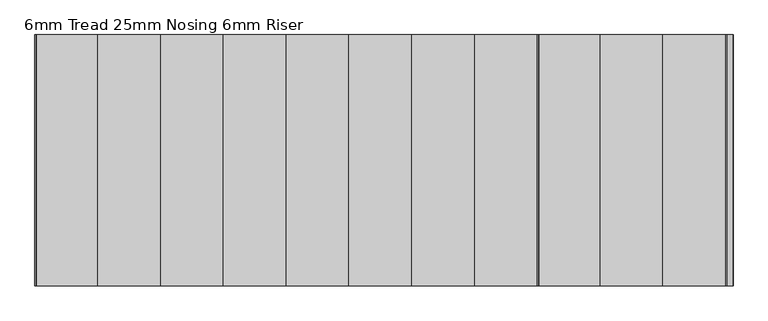
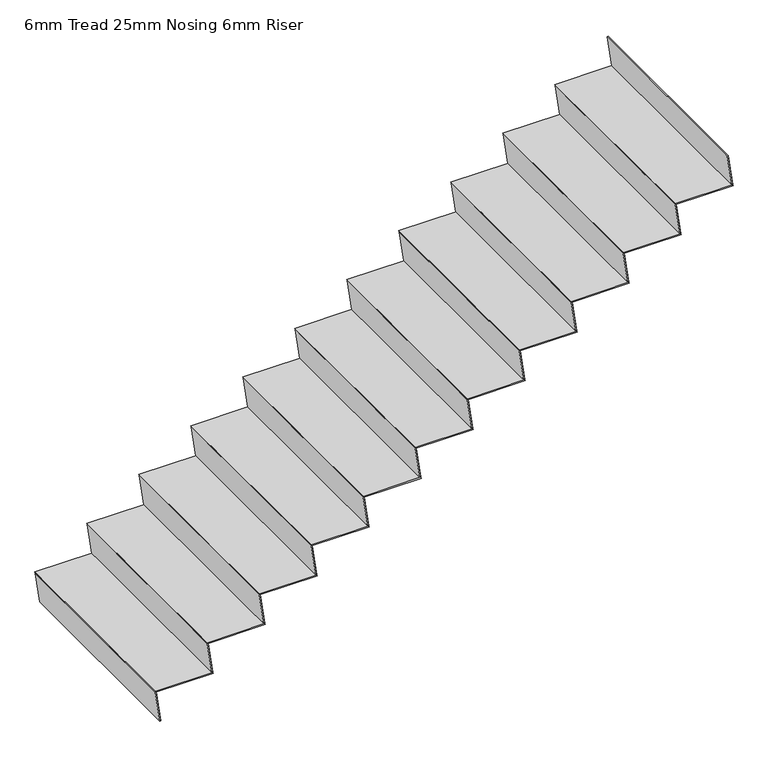
"""IFC4 building model written with IfcOpenShell, lengths in millimetres: stair flight geometry, 6mm Tread 25mm Nosing 6mm Riser."""

from ifc_helpers import new_model, si_unit, origin, place, context, project, spatial, faceted_brep, source, transform, mapped, element, save


def stair_flight_6mm_tread_25mm_nosing_6mm_riser_6b1513e0(model_context):
    return source(origin(), model_context, "Body", "Brep", [
        faceted_brep([(-16043.9400908, 12075.4345331, 22294.1176471), (-16043.0900908, 12075.4345331, 22288.1176471), (-16043.0900908, 13175.4345331, 22288.1176471), (-16043.9400908, 13175.4345331, 22294.1176471), (-16350.0, 13175.4345331, 22294.1176471), (-16350.0, 12075.4345331, 22294.1176471), (-16349.15, 12075.4345331, 22288.1176471), (-16349.15, 13175.4345331, 22288.1176471)], [[[0, 1, 2, 3]], [[3, 4, 5, 0]], [[2, 1, 6, 7]], [[4, 3, 2, 7]], [[0, 5, 6, 1]], [[5, 4, 7, 6]]]),
        faceted_brep([(-16349.15, 12075.4345331, 22288.1176471), (-16325.0, 12075.4345331, 22117.6470588), (-16318.9400908, 12075.4345331, 22117.6470588), (-16343.0900908, 12075.4345331, 22288.1176471), (-16349.15, 13175.4345331, 22288.1176471), (-16343.0900908, 13175.4345331, 22288.1176471), (-16318.9400908, 13175.4345331, 22117.6470588), (-16325.0, 13175.4345331, 22117.6470588)], [[[0, 1, 2, 3]], [[4, 5, 6, 7]], [[1, 0, 4, 7]], [[2, 1, 7, 6]], [[3, 2, 6, 5]], [[0, 3, 5, 4]]]),
        faceted_brep([(-16074.15, 12075.4345331, 22464.5882353), (-16050.0, 12075.4345331, 22294.1176471), (-16043.9400908, 12075.4345331, 22294.1176471), (-16068.0900908, 12075.4345331, 22464.5882353), (-16074.15, 13175.4345331, 22464.5882353), (-16068.0900908, 13175.4345331, 22464.5882353), (-16043.9400908, 13175.4345331, 22294.1176471), (-16050.0, 13175.4345331, 22294.1176471)], [[[0, 1, 2, 3]], [[4, 5, 6, 7]], [[1, 0, 4, 7]], [[2, 1, 7, 6]], [[3, 2, 6, 5]], [[0, 3, 5, 4]]]),
        faceted_brep([(-15768.9400908, 13175.4345331, 22470.5882353), (-16075.0, 13175.4345331, 22470.5882353), (-16075.0, 12075.4345331, 22470.5882353), (-15768.9400908, 12075.4345331, 22470.5882353), (-15768.0900908, 13175.4345331, 22464.5882353), (-15768.0900908, 12075.4345331, 22464.5882353), (-16074.15, 12075.4345331, 22464.5882353), (-16074.15, 13175.4345331, 22464.5882353)], [[[0, 1, 2, 3]], [[4, 5, 6, 7]], [[1, 0, 4, 7]], [[3, 2, 6, 5]], [[3, 5, 4, 0]], [[2, 1, 7, 6]]]),
        faceted_brep([(-15799.15, 12075.4345331, 22641.0588235), (-15775.0, 12075.4345331, 22470.5882353), (-15768.9400908, 12075.4345331, 22470.5882353), (-15793.0900908, 12075.4345331, 22641.0588235), (-15799.15, 13175.4345331, 22641.0588235), (-15793.0900908, 13175.4345331, 22641.0588235), (-15768.9400908, 13175.4345331, 22470.5882353), (-15775.0, 13175.4345331, 22470.5882353)], [[[0, 1, 2, 3]], [[4, 5, 6, 7]], [[1, 0, 4, 7]], [[2, 1, 7, 6]], [[3, 2, 6, 5]], [[0, 3, 5, 4]]]),
        faceted_brep([(-15493.9400908, 13175.4345331, 22647.0588235), (-15800.0, 13175.4345331, 22647.0588235), (-15800.0, 12075.4345331, 22647.0588235), (-15493.9400908, 12075.4345331, 22647.0588235), (-15493.0900908, 13175.4345331, 22641.0588235), (-15493.0900908, 12075.4345331, 22641.0588235), (-15799.15, 12075.4345331, 22641.0588235), (-15799.15, 13175.4345331, 22641.0588235)], [[[0, 1, 2, 3]], [[4, 5, 6, 7]], [[1, 0, 4, 7]], [[3, 2, 6, 5]], [[3, 5, 4, 0]], [[2, 1, 7, 6]]]),
        faceted_brep([(-15524.15, 12075.4345331, 22817.5294118), (-15500.0, 12075.4345331, 22647.0588235), (-15493.9400908, 12075.4345331, 22647.0588235), (-15518.0900908, 12075.4345331, 22817.5294118), (-15524.15, 13175.4345331, 22817.5294118), (-15518.0900908, 13175.4345331, 22817.5294118), (-15493.9400908, 13175.4345331, 22647.0588235), (-15500.0, 13175.4345331, 22647.0588235)], [[[0, 1, 2, 3]], [[4, 5, 6, 7]], [[1, 0, 4, 7]], [[2, 1, 7, 6]], [[3, 2, 6, 5]], [[0, 3, 5, 4]]]),
        faceted_brep([(-15218.9400908, 13175.4345331, 22823.5294118), (-15525.0, 13175.4345331, 22823.5294118), (-15525.0, 12075.4345331, 22823.5294118), (-15218.9400908, 12075.4345331, 22823.5294118), (-15218.0900908, 13175.4345331, 22817.5294118), (-15218.0900908, 12075.4345331, 22817.5294118), (-15524.15, 12075.4345331, 22817.5294118), (-15524.15, 13175.4345331, 22817.5294118)], [[[0, 1, 2, 3]], [[4, 5, 6, 7]], [[1, 0, 4, 7]], [[3, 2, 6, 5]], [[3, 5, 4, 0]], [[2, 1, 7, 6]]]),
        faceted_brep([(-15249.15, 12075.4345331, 22994.0), (-15225.0, 12075.4345331, 22823.5294118), (-15218.9400908, 12075.4345331, 22823.5294118), (-15243.0900908, 12075.4345331, 22994.0), (-15249.15, 13175.4345331, 22994.0), (-15243.0900908, 13175.4345331, 22994.0), (-15218.9400908, 13175.4345331, 22823.5294118), (-15225.0, 13175.4345331, 22823.5294118)], [[[0, 1, 2, 3]], [[4, 5, 6, 7]], [[1, 0, 4, 7]], [[2, 1, 7, 6]], [[3, 2, 6, 5]], [[0, 3, 5, 4]]]),
        faceted_brep([(-14943.9400908, 13175.4345331, 23000.0), (-15250.0, 13175.4345331, 23000.0), (-15250.0, 12075.4345331, 23000.0), (-14943.9400908, 12075.4345331, 23000.0), (-14943.0900908, 13175.4345331, 22994.0), (-14943.0900908, 12075.4345331, 22994.0), (-15249.15, 12075.4345331, 22994.0), (-15249.15, 13175.4345331, 22994.0)], [[[0, 1, 2, 3]], [[4, 5, 6, 7]], [[1, 0, 4, 7]], [[3, 2, 6, 5]], [[3, 5, 4, 0]], [[2, 1, 7, 6]]]),
        faceted_brep([(-14974.15, 12075.4345331, 23170.4705882), (-14950.0, 12075.4345331, 23000.0), (-14943.9400908, 12075.4345331, 23000.0), (-14968.0900908, 12075.4345331, 23170.4705882), (-14974.15, 13175.4345331, 23170.4705882), (-14968.0900908, 13175.4345331, 23170.4705882), (-14943.9400908, 13175.4345331, 23000.0), (-14950.0, 13175.4345331, 23000.0)], [[[0, 1, 2, 3]], [[4, 5, 6, 7]], [[1, 0, 4, 7]], [[2, 1, 7, 6]], [[3, 2, 6, 5]], [[0, 3, 5, 4]]]),
        faceted_brep([(-14668.9400908, 13175.4345331, 23176.4705882), (-14975.0, 13175.4345331, 23176.4705882), (-14975.0, 12075.4345331, 23176.4705882), (-14668.9400908, 12075.4345331, 23176.4705882), (-14668.0900908, 13175.4345331, 23170.4705882), (-14668.0900908, 12075.4345331, 23170.4705882), (-14974.15, 12075.4345331, 23170.4705882), (-14974.15, 13175.4345331, 23170.4705882)], [[[0, 1, 2, 3]], [[4, 5, 6, 7]], [[1, 0, 4, 7]], [[3, 2, 6, 5]], [[3, 5, 4, 0]], [[2, 1, 7, 6]]]),
        faceted_brep([(-14699.15, 12075.4345331, 23346.9411765), (-14675.0, 12075.4345331, 23176.4705882), (-14668.9400908, 12075.4345331, 23176.4705882), (-14693.0900908, 12075.4345331, 23346.9411765), (-14699.15, 13175.4345331, 23346.9411765), (-14693.0900908, 13175.4345331, 23346.9411765), (-14668.9400908, 13175.4345331, 23176.4705882), (-14675.0, 13175.4345331, 23176.4705882)], [[[0, 1, 2, 3]], [[4, 5, 6, 7]], [[1, 0, 4, 7]], [[2, 1, 7, 6]], [[3, 2, 6, 5]], [[0, 3, 5, 4]]]),
        faceted_brep([(-14393.9400908, 13175.4345331, 23352.9411765), (-14700.0, 13175.4345331, 23352.9411765), (-14700.0, 12075.4345331, 23352.9411765), (-14393.9400908, 12075.4345331, 23352.9411765), (-14393.0900908, 13175.4345331, 23346.9411765), (-14393.0900908, 12075.4345331, 23346.9411765), (-14699.15, 12075.4345331, 23346.9411765), (-14699.15, 13175.4345331, 23346.9411765)], [[[0, 1, 2, 3]], [[4, 5, 6, 7]], [[1, 0, 4, 7]], [[3, 2, 6, 5]], [[3, 5, 4, 0]], [[2, 1, 7, 6]]]),
        faceted_brep([(-14424.15, 12075.4345331, 23523.4117647), (-14400.0, 12075.4345331, 23352.9411765), (-14393.9400908, 12075.4345331, 23352.9411765), (-14418.0900908, 12075.4345331, 23523.4117647), (-14424.15, 13175.4345331, 23523.4117647), (-14418.0900908, 13175.4345331, 23523.4117647), (-14393.9400908, 13175.4345331, 23352.9411765), (-14400.0, 13175.4345331, 23352.9411765)], [[[0, 1, 2, 3]], [[4, 5, 6, 7]], [[1, 0, 4, 7]], [[2, 1, 7, 6]], [[3, 2, 6, 5]], [[0, 3, 5, 4]]]),
        faceted_brep([(-14118.9400908, 13175.4345331, 23529.4117647), (-14425.0, 13175.4345331, 23529.4117647), (-14425.0, 12075.4345331, 23529.4117647), (-14118.9400908, 12075.4345331, 23529.4117647), (-14118.0900908, 13175.4345331, 23523.4117647), (-14118.0900908, 12075.4345331, 23523.4117647), (-14424.15, 12075.4345331, 23523.4117647), (-14424.15, 13175.4345331, 23523.4117647)], [[[0, 1, 2, 3]], [[4, 5, 6, 7]], [[1, 0, 4, 7]], [[3, 2, 6, 5]], [[3, 5, 4, 0]], [[2, 1, 7, 6]]]),
        faceted_brep([(-14149.15, 12075.4345331, 23699.8823529), (-14125.0, 12075.4345331, 23529.4117647), (-14118.9400908, 12075.4345331, 23529.4117647), (-14143.0900908, 12075.4345331, 23699.8823529), (-14149.15, 13175.4345331, 23699.8823529), (-14143.0900908, 13175.4345331, 23699.8823529), (-14118.9400908, 13175.4345331, 23529.4117647), (-14125.0, 13175.4345331, 23529.4117647)], [[[0, 1, 2, 3]], [[4, 5, 6, 7]], [[1, 0, 4, 7]], [[2, 1, 7, 6]], [[3, 2, 6, 5]], [[0, 3, 5, 4]]]),
        faceted_brep([(-13843.9400908, 13175.4345331, 23705.8823529), (-14150.0, 13175.4345331, 23705.8823529), (-14150.0, 12075.4345331, 23705.8823529), (-13843.9400908, 12075.4345331, 23705.8823529), (-13843.0900908, 13175.4345331, 23699.8823529), (-13843.0900908, 12075.4345331, 23699.8823529), (-14149.15, 12075.4345331, 23699.8823529), (-14149.15, 13175.4345331, 23699.8823529)], [[[0, 1, 2, 3]], [[4, 5, 6, 7]], [[1, 0, 4, 7]], [[3, 2, 6, 5]], [[3, 5, 4, 0]], [[2, 1, 7, 6]]]),
        faceted_brep([(-13874.15, 12075.4345331, 23876.3529412), (-13850.0, 12075.4345331, 23705.8823529), (-13843.9400908, 12075.4345331, 23705.8823529), (-13868.0900908, 12075.4345331, 23876.3529412), (-13874.15, 13175.4345331, 23876.3529412), (-13868.0900908, 13175.4345331, 23876.3529412), (-13843.9400908, 13175.4345331, 23705.8823529), (-13850.0, 13175.4345331, 23705.8823529)], [[[0, 1, 2, 3]], [[4, 5, 6, 7]], [[1, 0, 4, 7]], [[2, 1, 7, 6]], [[3, 2, 6, 5]], [[0, 3, 5, 4]]]),
        faceted_brep([(-13568.9400908, 13175.4345331, 23882.3529412), (-13875.0, 13175.4345331, 23882.3529412), (-13875.0, 12075.4345331, 23882.3529412), (-13568.9400908, 12075.4345331, 23882.3529412), (-13568.0900908, 13175.4345331, 23876.3529412), (-13568.0900908, 12075.4345331, 23876.3529412), (-13874.15, 12075.4345331, 23876.3529412), (-13874.15, 13175.4345331, 23876.3529412)], [[[0, 1, 2, 3]], [[4, 5, 6, 7]], [[1, 0, 4, 7]], [[3, 2, 6, 5]], [[3, 5, 4, 0]], [[2, 1, 7, 6]]]),
        faceted_brep([(-13324.15, 12075.4345331, 24229.2941176), (-13300.0, 12075.4345331, 24058.8235294), (-13293.9400908, 12075.4345331, 24058.8235294), (-13318.0900908, 12075.4345331, 24229.2941176), (-13324.15, 13175.4345331, 24229.2941176), (-13318.0900908, 13175.4345331, 24229.2941176), (-13293.9400908, 13175.4345331, 24058.8235294), (-13300.0, 13175.4345331, 24058.8235294)], [[[0, 1, 2, 3]], [[4, 5, 6, 7]], [[1, 0, 4, 7]], [[2, 1, 7, 6]], [[3, 2, 6, 5]], [[0, 3, 5, 4]]]),
        faceted_brep([(-13599.15, 12075.4345331, 24052.8235294), (-13575.0, 12075.4345331, 23882.3529412), (-13568.9400908, 12075.4345331, 23882.3529412), (-13593.0900908, 12075.4345331, 24052.8235294), (-13599.15, 13175.4345331, 24052.8235294), (-13593.0900908, 13175.4345331, 24052.8235294), (-13568.9400908, 13175.4345331, 23882.3529412), (-13575.0, 13175.4345331, 23882.3529412)], [[[0, 1, 2, 3]], [[4, 5, 6, 7]], [[1, 0, 4, 7]], [[2, 1, 7, 6]], [[3, 2, 6, 5]], [[0, 3, 5, 4]]]),
        faceted_brep([(-13293.9400908, 13175.4345331, 24058.8235294), (-13325.0, 13175.4345331, 24058.8235294), (-13600.0, 13175.4345331, 24058.8235294), (-13600.0, 12075.4345331, 24058.8235294), (-13293.9400908, 12075.4345331, 24058.8235294), (-13293.0900908, 13175.4345331, 24052.8235294), (-13293.0900908, 12075.4345331, 24052.8235294), (-13599.15, 12075.4345331, 24052.8235294), (-13599.15, 13175.4345331, 24052.8235294), (-13325.0, 13175.4345331, 24052.8235294)], [[[0, 1, 2, 3, 4]], [[5, 6, 7, 8, 9]], [[1, 0, 5, 9]], [[2, 1, 9, 8]], [[4, 3, 7, 6]], [[4, 6, 5, 0]], [[3, 2, 8, 7]]]),
    ])


if __name__ == "__main__":
    model = new_model("IFC4")
    model_context = context("Model", 3, world=origin())
    ifc_project = project(units=[si_unit("LENGTHUNIT", "METRE", prefix="MILLI")], contexts=[model_context])
    site = spatial("IfcSite", under=ifc_project)
    building = spatial("IfcBuilding", under=site)
    placement = place(None, origin())
    stair_flight_6mm_tread_25mm_nosing_6mm_riser_shape = stair_flight_6mm_tread_25mm_nosing_6mm_riser_6b1513e0(model_context)
    element("IfcStairFlight", 1, ObjectType="6mm Tread 25mm Nosing 6mm Riser", at=placement, inside=building, context=model_context, shape_type="MappedRepresentation", body=[
        mapped(stair_flight_6mm_tread_25mm_nosing_6mm_riser_shape, transform((0.0, 0.0, 0.0), x_axis=(1.0, 0.0, 0.0), y_axis=(0.0, 1.0, 0.0), z_axis=(0.0, 0.0, 1.0))),
    ])
    save(model, "model.ifc")

# Revit data of these elements
# Element 1 (IfcStairFlight, "6mm Tread 25mm Nosing 6mm Riser")
#   Materials on its faces: "Steel, Paint Finish, Dark Gray"
# Materials
#   "Steel, Paint Finish, Dark Gray": class "Metal", colour RGB 89 89 89, transparency 0, Description = "Steel, paint finish, dark gray, glossy", Cost = 0
